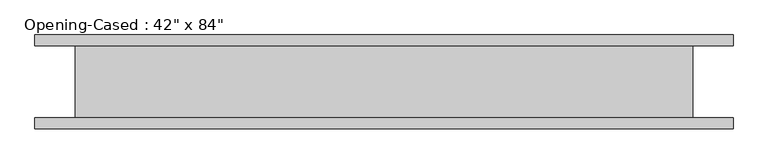
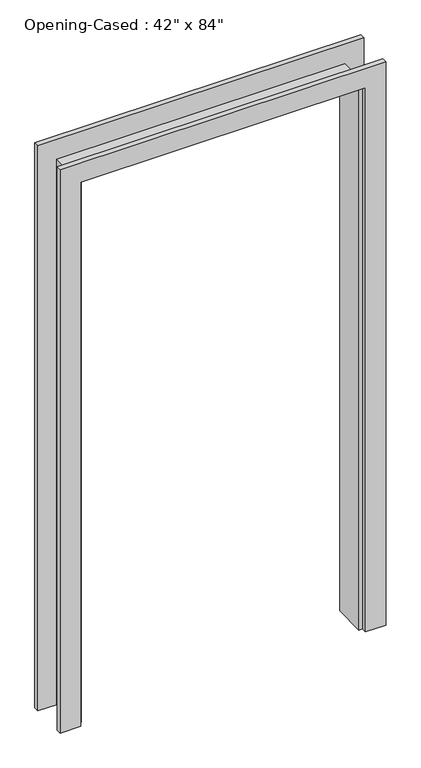
"""IFC4 building model written with IfcOpenShell, lengths in millimetres: proxy geometry."""

import ifcopenshell
import ifcopenshell.guid

model = None  # the IFC model being written
_history = None  # IfcOwnerHistory: only IFC2X3 demands one
_inside = {}  # id of a spatial element -> (the spatial element, [elements in it])
_under = {}  # id of a project, library or spatial element -> (it, [spatial elements below it])
_declared = {}  # id of a project -> (the project, [libraries it declares])
_typed = {}  # id of a type object -> (the type object, [elements of that type])
_made_of = {}  # id of a material, layer set ... -> (it, [elements and type objects made of it])


def new_model(schema):
    """Start an empty IFC model of exactly this schema.

    Asked for "IFC4X3", IfcOpenShell would pick the latest addendum, in which some entities
    have other attributes; the version numbers below select the first issue.
    IFC2X3 requires an IfcOwnerHistory on every rooted entity: one is made here for all.
    """
    global model, _history
    if schema == "IFC4X3":
        model = ifcopenshell.file(schema_version=(4, 3, 0, 0))
    else:
        model = ifcopenshell.file(schema=schema)
    _inside.clear()
    _under.clear()
    _declared.clear()
    _typed.clear()
    _made_of.clear()
    _history = None
    if model.schema == "IFC2X3":
        org = make("IfcOrganization", Name="unknown")
        user = make(
            "IfcPersonAndOrganization",
            ThePerson=make("IfcPerson", FamilyName="unknown"),
            TheOrganization=org,
        )
        app = make(
            "IfcApplication",
            ApplicationDeveloper=org,
            Version="unknown",
            ApplicationFullName="unknown",
            ApplicationIdentifier="unknown",
        )
        _history = make(
            "IfcOwnerHistory",
            OwningUser=user,
            OwningApplication=app,
            ChangeAction="ADDED",
            CreationDate=0,
        )
    return model


def make(cls, **values):
    """One entity of the class cls with the attributes given. An attribute that is None is left unset."""
    return model.create_entity(
        cls, **{name: value for name, value in values.items() if value is not None}
    )


def rooted(cls, **values):
    """An entity with a GlobalId (a new one), such as an element, a storey or a relation."""
    return make(cls, GlobalId=ifcopenshell.guid.new(), OwnerHistory=_history, **values)


def si_unit(unit_type, name, prefix=None):
    """IfcSIUnit, for example si_unit("LENGTHUNIT", "METRE", prefix="MILLI")."""
    return make("IfcSIUnit", UnitType=unit_type, Prefix=prefix, Name=name)


def assignment(units):
    """IfcUnitAssignment: the units of a project."""
    return None if units is None else make("IfcUnitAssignment", Units=units)


def point(xyz):
    """IfcCartesianPoint."""
    return None if xyz is None else make("IfcCartesianPoint", Coordinates=xyz)


def direction(xyz):
    """IfcDirection."""
    return None if xyz is None else make("IfcDirection", DirectionRatios=xyz)


def frame(location, z_axis=None, x_axis=None):
    """IfcAxis2Placement3D, a coordinate frame: its origin and axes. An axis left out is left unset."""
    return make(
        "IfcAxis2Placement3D",
        Location=point(location),
        Axis=direction(z_axis),
        RefDirection=direction(x_axis),
    )


def origin():
    """The frame at (0, 0, 0) with its axes left unset."""
    return frame((0.0, 0.0, 0.0))


def place(relative_to, where):
    """IfcLocalPlacement: puts the frame where relative to a parent placement (None: the world)."""
    return make(
        "IfcLocalPlacement", PlacementRelTo=relative_to, RelativePlacement=where
    )


def context(
    kind, dimensions, precision=None, world=None, true_north=None, identifier=None
):
    """IfcGeometricRepresentationContext, for example the 3D "Model" context."""
    return make(
        "IfcGeometricRepresentationContext",
        ContextIdentifier=identifier,
        ContextType=kind,
        CoordinateSpaceDimension=dimensions,
        Precision=precision,
        WorldCoordinateSystem=world,
        TrueNorth=true_north,
    )


def project(units=None, contexts=None):
    """IfcProject with its units and contexts."""
    return rooted(
        "IfcProject",
        Name="project",
        RepresentationContexts=contexts,
        UnitsInContext=assignment(units),
    )


def spatial(cls, under=None, at=None, **own):
    """A site, building, storey or space (cls), placed at a placement, below another one or the project."""
    s = rooted(cls, ObjectPlacement=at, **own)
    if under is not None:
        _under.setdefault(under.id(), (under, []))[1].append(s)
    return s


def polyline(points):
    """IfcPolyline through the points."""
    return make("IfcPolyline", Points=[point(p) for p in points])


def outline(outer, holes=None, kind="AREA"):
    """IfcArbitraryClosedProfileDef: a profile drawn as a closed curve; with holes, ...WithVoids."""
    if holes is None:
        return make("IfcArbitraryClosedProfileDef", ProfileType=kind, OuterCurve=outer)
    return make(
        "IfcArbitraryProfileDefWithVoids",
        ProfileType=kind,
        OuterCurve=outer,
        InnerCurves=holes,
    )


def extrude(swept, where, along, depth):
    """IfcExtrudedAreaSolid: the profile swept, set in the frame where, extruded along a direction by depth."""
    return make(
        "IfcExtrudedAreaSolid",
        SweptArea=swept,
        Position=where,
        ExtrudedDirection=direction(along),
        Depth=depth,
    )


def faces_of(points, faces, orient=None, outer=None):
    """IfcFace entities. A face is a list of loops; a loop is a list of indices into points, from 0.

    orient and outer hold one flag for each loop. By default every Orientation is true, the
    first loop of a face is its IfcFaceOuterBound and the others are IfcFaceBound.
    """
    made = []
    for i, loops in enumerate(faces):
        bounds = []
        for j, loop in enumerate(loops):
            is_outer = j == 0 if outer is None else outer[i][j]
            bounds.append(
                make(
                    "IfcFaceOuterBound" if is_outer else "IfcFaceBound",
                    Bound=make("IfcPolyLoop", Polygon=[points[k] for k in loop]),
                    Orientation=True if orient is None else orient[i][j],
                )
            )
        made.append(make("IfcFace", Bounds=bounds))
    return made


def faceted_brep(points, faces, orient=None, outer=None, voids=None):
    """IfcFacetedBrep: a solid bounded by flat faces; with voids (closed shells), ...WithVoids."""
    shared = [point(p) for p in points]
    hull = make("IfcClosedShell", CfsFaces=faces_of(shared, faces, orient, outer))
    if voids is None:
        return make("IfcFacetedBrep", Outer=hull)
    return make(
        "IfcFacetedBrepWithVoids",
        Outer=hull,
        Voids=[
            make(cls, CfsFaces=faces_of(shared, fs, o, b)) for cls, fs, o, b in voids
        ],
    )


def shape(context_of_items, identifier, shape_type, items):
    """IfcShapeRepresentation: the items that make up one representation, for example the "Body"."""
    return make(
        "IfcShapeRepresentation",
        ContextOfItems=context_of_items,
        RepresentationIdentifier=identifier,
        RepresentationType=shape_type,
        Items=items,
    )


def source(mapping_origin, context_of_items, identifier, shape_type, items):
    """IfcRepresentationMap: a shape defined once, which mapped items show again and again."""
    return make(
        "IfcRepresentationMap",
        MappingOrigin=mapping_origin,
        MappedRepresentation=shape(context_of_items, identifier, shape_type, items),
    )


def transform(
    local_origin,
    x_axis=None,
    y_axis=None,
    z_axis=None,
    scale=None,
    scale2=None,
    scale3=None,
    uniform=True,
):
    """IfcCartesianTransformationOperator3D, or its non-uniform kind. x_axis, y_axis, z_axis: its Axis1, 2, 3."""
    if uniform:
        return make(
            "IfcCartesianTransformationOperator3D",
            Axis1=direction(x_axis),
            Axis2=direction(y_axis),
            LocalOrigin=point(local_origin),
            Scale=scale,
            Axis3=direction(z_axis),
        )
    return make(
        "IfcCartesianTransformationOperator3DnonUniform",
        Axis1=direction(x_axis),
        Axis2=direction(y_axis),
        LocalOrigin=point(local_origin),
        Scale=scale,
        Axis3=direction(z_axis),
        Scale2=scale2,
        Scale3=scale3,
    )


def mapped(mapping_source, mapping_target):
    """IfcMappedItem: shows the shape of a source again, moved by a transform."""
    return make(
        "IfcMappedItem", MappingSource=mapping_source, MappingTarget=mapping_target
    )


def made_of(thing, what):
    """Note that an element or type object is made of a material, layer set ...; save() writes the relation."""
    if what is not None:
        _made_of.setdefault(what.id(), (what, []))[1].append(thing)
    return thing


def element(
    cls,
    number,
    at=None,
    inside=None,
    cuts=None,
    type_object=None,
    material=None,
    context=None,
    identifier="Body",
    shape_type=None,
    held_by="IfcProductDefinitionShape",
    body=None,
    shapes=None,
    **own,
):
    """One element of the class cls, such as IfcWall. Its Tag is "e" and its number.

    at: its placement. inside: the storey or other place that contains it. cuts: it is an
    opening in that element (IfcRelVoidsElement). A single representation is given by context,
    identifier, shape_type and body (its items); several are given by shapes. held_by: the class
    of the entity that holds the representations. save() writes the other relations.
    """
    e = rooted(cls, Tag="e%d" % number, ObjectPlacement=at, **own)
    if body is not None:
        shapes = [shape(context, identifier, shape_type, body)]
    if shapes is not None:
        e.Representation = make(held_by, Representations=shapes)
    if inside is not None:
        _inside.setdefault(inside.id(), (inside, []))[1].append(e)
    if cuts is not None:
        rooted(
            "IfcRelVoidsElement", RelatingBuildingElement=cuts, RelatedOpeningElement=e
        )
    if type_object is not None:
        _typed.setdefault(type_object.id(), (type_object, []))[1].append(e)
    return made_of(e, material)


def aggregate(whole, parts):
    """IfcRelAggregates: a whole, such as a stair, and the parts it consists of."""
    return rooted("IfcRelAggregates", RelatingObject=whole, RelatedObjects=parts)


def save(model, path):
    """Write the relations noted so far, then the file.

    IfcRelAggregates (storeys below a building ...), IfcRelContainedInSpatialStructure (elements
    in a storey), IfcRelDefinesByType, IfcRelAssociatesMaterial and IfcRelDeclares: one each for
    every whole, place, type object, material and project.
    """
    for whole, parts in _under.values():
        aggregate(whole, parts)
    for where, things in _inside.values():
        rooted(
            "IfcRelContainedInSpatialStructure",
            RelatedElements=things,
            RelatingStructure=where,
        )
    for kind, things in _typed.values():
        rooted("IfcRelDefinesByType", RelatedObjects=things, RelatingType=kind)
    for what, things in _made_of.values():
        rooted("IfcRelAssociatesMaterial", RelatedObjects=things, RelatingMaterial=what)
    for by, libraries in _declared.values():
        rooted("IfcRelDeclares", RelatingContext=by, RelatedDefinitions=libraries)
    model.write(path)


def proxy_de02396b(model_context):
    return source(origin(), model_context, "Body", "SolidModel", [
        faceted_brep([(506.1613433, 61.9125, 0.0), (525.2113433, 61.9125, 0.0), (525.2113433, -61.9125, 0.0), (506.1613433, -61.9125, 0.0), (506.1613433, 61.9125, 2114.55), (525.2113433, 61.9125, 2133.6), (525.2113433, -61.9125, 2133.6), (506.1613433, -61.9125, 2114.55), (-522.5386567, 61.9125, 2114.55), (-541.5886567, 61.9125, 2133.6), (-541.5886567, -61.9125, 2133.6), (-522.5386567, -61.9125, 2114.55), (-522.5386567, 61.9125, 0.0), (-522.5386567, -61.9125, 0.0), (-541.5886567, -61.9125, 0.0), (-541.5886567, 61.9125, 0.0)], [[[0, 1, 2, 3]], [[1, 0, 4, 5]], [[2, 1, 5, 6]], [[3, 2, 6, 7]], [[0, 3, 7, 4]], [[5, 4, 8, 9]], [[6, 5, 9, 10]], [[7, 6, 10, 11]], [[4, 7, 11, 8]], [[12, 13, 14, 15]], [[9, 8, 12, 15]], [[10, 9, 15, 14]], [[11, 10, 14, 13]], [[8, 11, 13, 12]]]),
        extrude(outline(polyline([(0.0, -535.2386567), (2127.25, -535.2386567), (2127.25, 518.8613433), (0.0, 518.8613433), (0.0, 595.0613433), (2203.45, 595.0613433), (2203.45, -611.4386567), (0.0, -611.4386567), (0.0, -535.2386567)])), frame((0.0, -80.9625, 0.0), z_axis=(0.0, 1.0, 0.0), x_axis=(0.0, 0.0, 1.0)), (0.0, 0.0, 1.0), 19.05),
        extrude(outline(polyline([(0.0, 595.0613433), (2209.8, 595.0613433), (2209.8, -611.4386567), (0.0, -611.4386567), (0.0, -535.2386567), (2127.25, -535.2386567), (2127.25, 518.8613433), (0.0, 518.8613433), (0.0, 595.0613433)])), frame((0.0, 61.9125, 0.0), z_axis=(0.0, 1.0, 0.0), x_axis=(0.0, 0.0, 1.0)), (0.0, 0.0, 1.0), 19.05),
    ])


if __name__ == "__main__":
    model = new_model("IFC4")
    model_context = context("Model", 3, world=origin())
    ifc_project = project(units=[si_unit("LENGTHUNIT", "METRE", prefix="MILLI")], contexts=[model_context])
    site = spatial("IfcSite", under=ifc_project)
    building = spatial("IfcBuilding", under=site)
    placement = place(None, origin())
    proxy_shape = proxy_de02396b(model_context)
    element("IfcBuildingElementProxy", 1, Name="Opening-Cased : 42\" x 84\"", ObjectType="Opening-Cased : 42\" x 84\"", at=placement, inside=building, context=model_context, shape_type="MappedRepresentation", body=[
        mapped(proxy_shape, transform((0.0, 0.0, 0.0), x_axis=(1.0, 0.0, 0.0), y_axis=(0.0, 1.0, 0.0), z_axis=(0.0, 0.0, 1.0))),
    ])
    save(model, "model.ifc")

# Revit data of these elements
# Project information
#   Room Abbreviation = "NBCD2"
#   Room Description = "Decontamination Shower (NBCD2)"
#   Sheets - Total = "6"
#   Project Issue Date = "Issue Date"
#   Project Status = "Project Status"
#   Client Name = "Owner"
#   Project Address = "Enter address here"
#   Project Name = "Project Name"
#   Project Number = "Project Number"
#   Publication Date = "30-Jan-15"
# Type "Opening-Cased : 42\" x 84\""
#   Height = 7' - 0"
#   Trim Thickness = 0' - 0 3/4"
#   Trim Width = 0' - 3"
#   Width = 3' - 6"
#   Frame Material = Door - Frame
# Element 1 (IfcBuildingElementProxy, "Opening-Cased : 42\" x 84\"")
#   Materials on its faces: "Door - Frame"
# Materials
#   "Door - Frame": class "Miscellaneous", colour RGB 118 70 51, transparency 0
